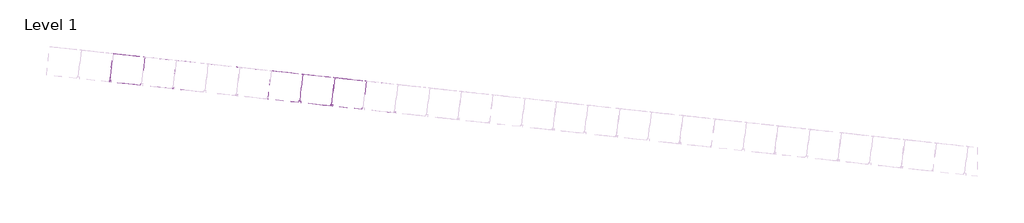
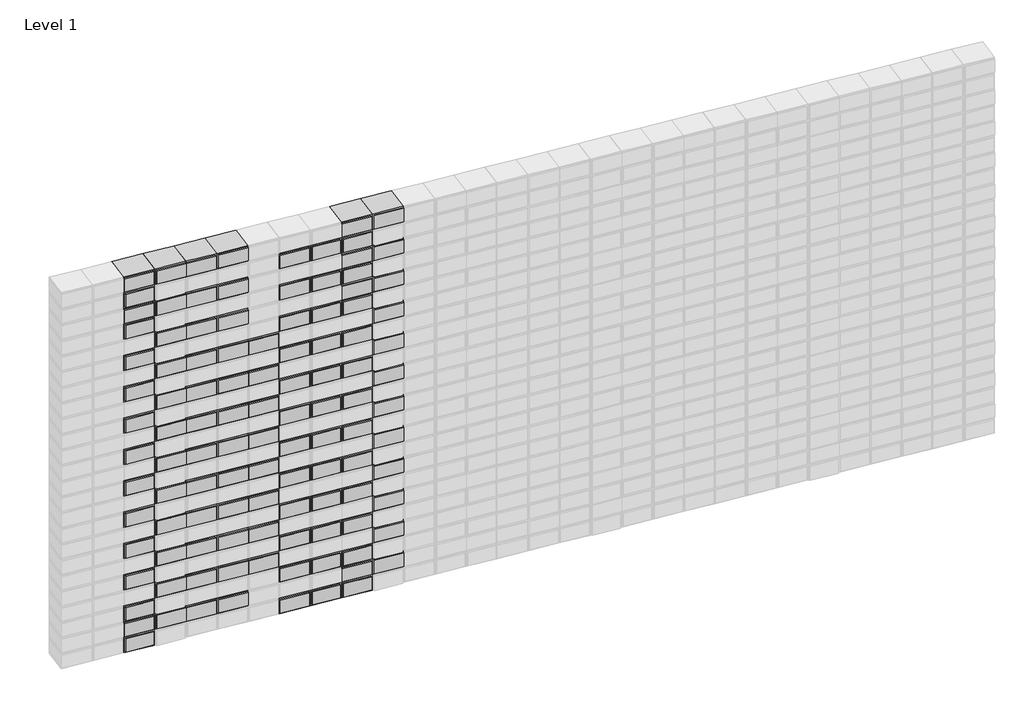
# One storey, part 12 of 18: 111 proxies.
"""IFC4 building model written with IfcOpenShell, lengths in millimetres."""

import ifcopenshell
import ifcopenshell.guid

model = None  # the IFC model being written
_history = None  # IfcOwnerHistory: only IFC2X3 demands one
_inside = {}  # id of a spatial element -> (the spatial element, [elements in it])
_under = {}  # id of a project, library or spatial element -> (it, [spatial elements below it])
_declared = {}  # id of a project -> (the project, [libraries it declares])
_typed = {}  # id of a type object -> (the type object, [elements of that type])
_made_of = {}  # id of a material, layer set ... -> (it, [elements and type objects made of it])


def new_model(schema):
    """Start an empty IFC model of exactly this schema.

    Asked for "IFC4X3", IfcOpenShell would pick the latest addendum, in which some entities
    have other attributes; the version numbers below select the first issue.
    IFC2X3 requires an IfcOwnerHistory on every rooted entity: one is made here for all.
    """
    global model, _history
    if schema == "IFC4X3":
        model = ifcopenshell.file(schema_version=(4, 3, 0, 0))
    else:
        model = ifcopenshell.file(schema=schema)
    _inside.clear()
    _under.clear()
    _declared.clear()
    _typed.clear()
    _made_of.clear()
    _history = None
    if model.schema == "IFC2X3":
        org = make("IfcOrganization", Name="unknown")
        user = make(
            "IfcPersonAndOrganization",
            ThePerson=make("IfcPerson", FamilyName="unknown"),
            TheOrganization=org,
        )
        app = make(
            "IfcApplication",
            ApplicationDeveloper=org,
            Version="unknown",
            ApplicationFullName="unknown",
            ApplicationIdentifier="unknown",
        )
        _history = make(
            "IfcOwnerHistory",
            OwningUser=user,
            OwningApplication=app,
            ChangeAction="ADDED",
            CreationDate=0,
        )
    return model


def make(cls, **values):
    """One entity of the class cls with the attributes given. An attribute that is None is left unset."""
    return model.create_entity(
        cls, **{name: value for name, value in values.items() if value is not None}
    )


def rooted(cls, **values):
    """An entity with a GlobalId (a new one), such as an element, a storey or a relation."""
    return make(cls, GlobalId=ifcopenshell.guid.new(), OwnerHistory=_history, **values)


def si_unit(unit_type, name, prefix=None):
    """IfcSIUnit, for example si_unit("LENGTHUNIT", "METRE", prefix="MILLI")."""
    return make("IfcSIUnit", UnitType=unit_type, Prefix=prefix, Name=name)


def assignment(units):
    """IfcUnitAssignment: the units of a project."""
    return None if units is None else make("IfcUnitAssignment", Units=units)


def point(xyz):
    """IfcCartesianPoint."""
    return None if xyz is None else make("IfcCartesianPoint", Coordinates=xyz)


def direction(xyz):
    """IfcDirection."""
    return None if xyz is None else make("IfcDirection", DirectionRatios=xyz)


def frame(location, z_axis=None, x_axis=None):
    """IfcAxis2Placement3D, a coordinate frame: its origin and axes. An axis left out is left unset."""
    return make(
        "IfcAxis2Placement3D",
        Location=point(location),
        Axis=direction(z_axis),
        RefDirection=direction(x_axis),
    )


def origin():
    """The frame at (0, 0, 0) with its axes left unset."""
    return frame((0.0, 0.0, 0.0))


def origin_with_axes():
    """The frame at (0, 0, 0) with the z axis (0, 0, 1) and the x axis (1, 0, 0) written out."""
    return frame((0.0, 0.0, 0.0), z_axis=(0.0, 0.0, 1.0), x_axis=(1.0, 0.0, 0.0))


def place(relative_to, where):
    """IfcLocalPlacement: puts the frame where relative to a parent placement (None: the world)."""
    return make(
        "IfcLocalPlacement", PlacementRelTo=relative_to, RelativePlacement=where
    )


def context(
    kind, dimensions, precision=None, world=None, true_north=None, identifier=None
):
    """IfcGeometricRepresentationContext, for example the 3D "Model" context."""
    return make(
        "IfcGeometricRepresentationContext",
        ContextIdentifier=identifier,
        ContextType=kind,
        CoordinateSpaceDimension=dimensions,
        Precision=precision,
        WorldCoordinateSystem=world,
        TrueNorth=true_north,
    )


def project(units=None, contexts=None):
    """IfcProject with its units and contexts."""
    return rooted(
        "IfcProject",
        Name="project",
        RepresentationContexts=contexts,
        UnitsInContext=assignment(units),
    )


def spatial(cls, under=None, at=None, **own):
    """A site, building, storey or space (cls), placed at a placement, below another one or the project."""
    s = rooted(cls, ObjectPlacement=at, **own)
    if under is not None:
        _under.setdefault(under.id(), (under, []))[1].append(s)
    return s


def polyline(points):
    """IfcPolyline through the points."""
    return make("IfcPolyline", Points=[point(p) for p in points])


def outline(outer, holes=None, kind="AREA"):
    """IfcArbitraryClosedProfileDef: a profile drawn as a closed curve; with holes, ...WithVoids."""
    if holes is None:
        return make("IfcArbitraryClosedProfileDef", ProfileType=kind, OuterCurve=outer)
    return make(
        "IfcArbitraryProfileDefWithVoids",
        ProfileType=kind,
        OuterCurve=outer,
        InnerCurves=holes,
    )


def extrude(swept, where, along, depth):
    """IfcExtrudedAreaSolid: the profile swept, set in the frame where, extruded along a direction by depth."""
    return make(
        "IfcExtrudedAreaSolid",
        SweptArea=swept,
        Position=where,
        ExtrudedDirection=direction(along),
        Depth=depth,
    )


def shape(context_of_items, identifier, shape_type, items):
    """IfcShapeRepresentation: the items that make up one representation, for example the "Body"."""
    return make(
        "IfcShapeRepresentation",
        ContextOfItems=context_of_items,
        RepresentationIdentifier=identifier,
        RepresentationType=shape_type,
        Items=items,
    )


def source(mapping_origin, context_of_items, identifier, shape_type, items):
    """IfcRepresentationMap: a shape defined once, which mapped items show again and again."""
    return make(
        "IfcRepresentationMap",
        MappingOrigin=mapping_origin,
        MappedRepresentation=shape(context_of_items, identifier, shape_type, items),
    )


def transform(
    local_origin,
    x_axis=None,
    y_axis=None,
    z_axis=None,
    scale=None,
    scale2=None,
    scale3=None,
    uniform=True,
):
    """IfcCartesianTransformationOperator3D, or its non-uniform kind. x_axis, y_axis, z_axis: its Axis1, 2, 3."""
    if uniform:
        return make(
            "IfcCartesianTransformationOperator3D",
            Axis1=direction(x_axis),
            Axis2=direction(y_axis),
            LocalOrigin=point(local_origin),
            Scale=scale,
            Axis3=direction(z_axis),
        )
    return make(
        "IfcCartesianTransformationOperator3DnonUniform",
        Axis1=direction(x_axis),
        Axis2=direction(y_axis),
        LocalOrigin=point(local_origin),
        Scale=scale,
        Axis3=direction(z_axis),
        Scale2=scale2,
        Scale3=scale3,
    )


def mapped(mapping_source, mapping_target):
    """IfcMappedItem: shows the shape of a source again, moved by a transform."""
    return make(
        "IfcMappedItem", MappingSource=mapping_source, MappingTarget=mapping_target
    )


def made_of(thing, what):
    """Note that an element or type object is made of a material, layer set ...; save() writes the relation."""
    if what is not None:
        _made_of.setdefault(what.id(), (what, []))[1].append(thing)
    return thing


def element(
    cls,
    number,
    at=None,
    inside=None,
    cuts=None,
    type_object=None,
    material=None,
    context=None,
    identifier="Body",
    shape_type=None,
    held_by="IfcProductDefinitionShape",
    body=None,
    shapes=None,
    **own,
):
    """One element of the class cls, such as IfcWall. Its Tag is "e" and its number.

    at: its placement. inside: the storey or other place that contains it. cuts: it is an
    opening in that element (IfcRelVoidsElement). A single representation is given by context,
    identifier, shape_type and body (its items); several are given by shapes. held_by: the class
    of the entity that holds the representations. save() writes the other relations.
    """
    e = rooted(cls, Tag="e%d" % number, ObjectPlacement=at, **own)
    if body is not None:
        shapes = [shape(context, identifier, shape_type, body)]
    if shapes is not None:
        e.Representation = make(held_by, Representations=shapes)
    if inside is not None:
        _inside.setdefault(inside.id(), (inside, []))[1].append(e)
    if cuts is not None:
        rooted(
            "IfcRelVoidsElement", RelatingBuildingElement=cuts, RelatedOpeningElement=e
        )
    if type_object is not None:
        _typed.setdefault(type_object.id(), (type_object, []))[1].append(e)
    return made_of(e, material)


def aggregate(whole, parts):
    """IfcRelAggregates: a whole, such as a stair, and the parts it consists of."""
    return rooted("IfcRelAggregates", RelatingObject=whole, RelatedObjects=parts)


def save(model, path):
    """Write the relations noted so far, then the file.

    IfcRelAggregates (storeys below a building ...), IfcRelContainedInSpatialStructure (elements
    in a storey), IfcRelDefinesByType, IfcRelAssociatesMaterial and IfcRelDeclares: one each for
    every whole, place, type object, material and project.
    """
    for whole, parts in _under.values():
        aggregate(whole, parts)
    for where, things in _inside.values():
        rooted(
            "IfcRelContainedInSpatialStructure",
            RelatedElements=things,
            RelatingStructure=where,
        )
    for kind, things in _typed.values():
        rooted("IfcRelDefinesByType", RelatedObjects=things, RelatingType=kind)
    for what, things in _made_of.values():
        rooted("IfcRelAssociatesMaterial", RelatedObjects=things, RelatingMaterial=what)
    for by, libraries in _declared.values():
        rooted("IfcRelDeclares", RelatingContext=by, RelatedDefinitions=libraries)
    model.write(path)


def geel_a5fc7152(model_context):
    return source(origin(), model_context, "Body", "SweptSolid", [
        extrude(outline(polyline([(131.1871262, 51.8695461), (24.8461542, 24.0369432), (23.5801491, 28.8740117), (125.0840527, 55.4406095), (111.9430518, 105.6488784), (10.4391482, 79.0822806), (9.1731432, 83.919349), (115.5141152, 111.7519519), (131.1871262, 51.8695461)])), origin_with_axes(), (0.0, 0.0, 1.0), 95.0),
        extrude(outline(polyline([(111.9430518, 105.6488784), (125.0840527, 55.4406095), (23.5801491, 28.8740117), (10.4391482, 79.0822806), (111.9430518, 105.6488784)])), origin_with_axes(), (0.0, 0.0, 1.0), 100.0),
    ])


def geel_ff5a4212(model_context):
    return source(origin(), model_context, "Body", "SweptSolid", [
        extrude(outline(polyline([(24.8461542, 24.0369432), (9.1731432, 83.919349), (115.5141152, 111.7519519), (116.7801202, 106.9148835), (15.2762167, 80.3482856), (28.4172176, 30.1400167), (129.9211211, 56.7066146), (131.1871262, 51.8695461), (24.8461542, 24.0369432)])), origin_with_axes(), (0.0, 0.0, 1.0), 95.0),
        extrude(outline(polyline([(116.7801202, 106.9148835), (129.9211211, 56.7066146), (28.4172176, 30.1400167), (15.2762167, 80.3482856), (116.7801202, 106.9148835)])), origin_with_axes(), (0.0, 0.0, 1.0), 100.0),
    ])


def rood_14a66368(model_context):
    return source(origin(), model_context, "Body", "SweptSolid", [
        extrude(outline(polyline([(24.8461542, 24.0369432), (9.1731432, 83.919349), (115.5141152, 111.7519519), (131.1871262, 51.8695461), (24.8461542, 24.0369432)]), holes=[polyline([(125.0840527, 55.4406095), (111.9430518, 105.6488784), (15.2762167, 80.3482856), (28.4172176, 30.1400167), (125.0840527, 55.4406095)])]), origin_with_axes(), (0.0, 0.0, 1.0), 95.0),
        extrude(outline(polyline([(111.9430518, 105.6488784), (125.0840527, 55.4406095), (28.4172176, 30.1400167), (15.2762167, 80.3482856), (111.9430518, 105.6488784)])), origin_with_axes(), (0.0, 0.0, 1.0), 100.0),
    ])


model = new_model("IFC4")

# Units and contexts
model_context = context("Model", 3, world=origin())
ifc_project = project(units=[si_unit("LENGTHUNIT", "METRE", prefix="MILLI")], contexts=[model_context])

# Site, building, storey
site = spatial("IfcSite", under=ifc_project)
building = spatial("IfcBuilding", under=site)
storey = spatial("IfcBuildingStorey", under=building, Name="Level 1", Elevation=0.0)

# Proxies
placement = place(None, origin())
geel_shape = geel_a5fc7152(model_context)
element("IfcBuildingElementProxy", 1, Name="Geel", ObjectType="Geel", at=placement, inside=storey, context=model_context, shape_type="MappedRepresentation", body=[
    mapped(geel_shape, transform((9860.5813726, -4383.3697112, 3159.1275502), x_axis=(0.9617275503729372, -0.1047347566147745, -0.2532010063378768), y_axis=(0.2517127736886921, -0.02741220845643024, 0.9674136914420256), z_axis=(-0.10826263628609285, -0.9941223272738547, 0.0))),
])
element("IfcBuildingElementProxy", 2, Name="Geel", ObjectType="Geel", at=placement, inside=storey, context=model_context, shape_type="MappedRepresentation", body=[
    mapped(geel_shape, transform((9095.6433234, -4300.0658686, 3282.926513), x_axis=(0.9617275503729401, -0.10473475661476903, -0.2532010063378687), y_axis=(0.2517127736886843, -0.02741220845642789, 0.9674136914420278), z_axis=(-0.108262636286087, -0.9941223272738555, 0.0))),
])
element("IfcBuildingElementProxy", 3, Name="Geel", ObjectType="Geel", at=placement, inside=storey, context=model_context, shape_type="MappedRepresentation", body=[
    mapped(geel_shape, transform((9860.5813726, -4383.3697112, 3282.926513), x_axis=(0.9617275503729372, -0.1047347566147745, -0.2532010063378768), y_axis=(0.2517127736886921, -0.02741220845643024, 0.9674136914420256), z_axis=(-0.10826263628609285, -0.9941223272738547, 0.0))),
])
element("IfcBuildingElementProxy", 4, Name="Geel", ObjectType="Geel", at=placement, inside=storey, context=model_context, shape_type="MappedRepresentation", body=[
    mapped(geel_shape, transform((9095.6433234, -4300.0658686, 3406.7254759), x_axis=(0.9617275503729401, -0.10473475661476903, -0.2532010063378687), y_axis=(0.2517127736886843, -0.02741220845642789, 0.9674136914420278), z_axis=(-0.108262636286087, -0.9941223272738555, 0.0))),
])
element("IfcBuildingElementProxy", 5, Name="Geel", ObjectType="Geel", at=placement, inside=storey, context=model_context, shape_type="MappedRepresentation", body=[
    mapped(geel_shape, transform((9860.5813726, -4383.3697112, 3406.7254759), x_axis=(0.9617275503729372, -0.1047347566147745, -0.2532010063378768), y_axis=(0.2517127736886921, -0.02741220845643024, 0.9674136914420256), z_axis=(-0.10826263628609285, -0.9941223272738547, 0.0))),
])
element("IfcBuildingElementProxy", 6, Name="Geel", ObjectType="Geel", at=placement, inside=storey, context=model_context, shape_type="MappedRepresentation", body=[
    mapped(geel_shape, transform((9095.6433234, -4300.0658686, 2044.9368847), x_axis=(0.961727550372941, -0.10473475661476911, -0.2532010063378651), y_axis=(0.2517127736886807, -0.0274122084564275, 0.9674136914420286), z_axis=(-0.10826263628608698, -0.9941223272738555, 0.0))),
])
element("IfcBuildingElementProxy", 7, Name="Geel", ObjectType="Geel", at=placement, inside=storey, context=model_context, shape_type="MappedRepresentation", body=[
    mapped(geel_shape, transform((9860.5813726, -4383.3697112, 2044.9368847), x_axis=(0.9617275503729381, -0.10473475661477456, -0.2532010063378731), y_axis=(0.2517127736886886, -0.02741220845642988, 0.9674136914420264), z_axis=(-0.10826263628609287, -0.9941223272738549, 0.0))),
])
element("IfcBuildingElementProxy", 8, Name="Geel", ObjectType="Geel", at=placement, inside=storey, context=model_context, shape_type="MappedRepresentation", body=[
    mapped(geel_shape, transform((9314.1970517, -4323.8669665, 2168.7358475), x_axis=(0.9617275503729396, -0.10473475661477374, -0.25320100633786874), y_axis=(0.251712773688684, -0.027412208456429103, 0.9674136914420278), z_axis=(-0.10826263628609185, -0.994122327273855, 0.0))),
])
element("IfcBuildingElementProxy", 9, Name="Geel", ObjectType="Geel", at=placement, inside=storey, context=model_context, shape_type="MappedRepresentation", body=[
    mapped(geel_shape, transform((9314.1970517, -4323.8669665, 2292.5348104), x_axis=(0.9617275503729396, -0.10473475661477374, -0.25320100633786874), y_axis=(0.251712773688684, -0.027412208456429103, 0.9674136914420278), z_axis=(-0.10826263628609185, -0.994122327273855, 0.0))),
])
element("IfcBuildingElementProxy", 10, Name="Geel", ObjectType="Geel", at=placement, inside=storey, context=model_context, shape_type="MappedRepresentation", body=[
    mapped(geel_shape, transform((9314.1970517, -4323.8669665, 2416.3337732), x_axis=(0.9617275503729403, -0.10473475661477383, -0.253201006337865), y_axis=(0.2517127736886804, -0.0274122084564287, 0.9674136914420286), z_axis=(-0.10826263628609184, -0.9941223272738549, 0.0))),
])
element("IfcBuildingElementProxy", 11, Name="Geel", ObjectType="Geel", at=placement, inside=storey, context=model_context, shape_type="MappedRepresentation", body=[
    mapped(geel_shape, transform((9314.1970517, -4323.8669665, 2540.132736), x_axis=(0.9617275503729396, -0.10473475661477374, -0.25320100633786874), y_axis=(0.251712773688684, -0.027412208456429103, 0.9674136914420278), z_axis=(-0.10826263628609185, -0.994122327273855, 0.0))),
])
element("IfcBuildingElementProxy", 12, Name="Geel", ObjectType="Geel", at=placement, inside=storey, context=model_context, shape_type="MappedRepresentation", body=[
    mapped(geel_shape, transform((9314.1970517, -4323.8669665, 2663.9316989), x_axis=(0.9617275503729396, -0.10473475661477374, -0.25320100633786874), y_axis=(0.251712773688684, -0.027412208456429103, 0.9674136914420278), z_axis=(-0.10826263628609185, -0.994122327273855, 0.0))),
])
element("IfcBuildingElementProxy", 13, Name="Geel", ObjectType="Geel", at=placement, inside=storey, context=model_context, shape_type="MappedRepresentation", body=[
    mapped(geel_shape, transform((9314.1970517, -4323.8669665, 2787.7306617), x_axis=(0.9617275503729396, -0.10473475661477374, -0.25320100633786874), y_axis=(0.251712773688684, -0.027412208456429103, 0.9674136914420278), z_axis=(-0.10826263628609185, -0.994122327273855, 0.0))),
])
element("IfcBuildingElementProxy", 14, Name="Geel", ObjectType="Geel", at=placement, inside=storey, context=model_context, shape_type="MappedRepresentation", body=[
    mapped(geel_shape, transform((9314.1970517, -4323.8669665, 2911.5296245), x_axis=(0.9617275503729396, -0.10473475661477374, -0.25320100633786874), y_axis=(0.251712773688684, -0.027412208456429103, 0.9674136914420278), z_axis=(-0.10826263628609185, -0.994122327273855, 0.0))),
])
element("IfcBuildingElementProxy", 15, Name="Geel", ObjectType="Geel", at=placement, inside=storey, context=model_context, shape_type="MappedRepresentation", body=[
    mapped(geel_shape, transform((9314.1970517, -4323.8669665, 3035.3285874), x_axis=(0.9617275503729396, -0.10473475661477374, -0.25320100633786874), y_axis=(0.251712773688684, -0.027412208456429103, 0.9674136914420278), z_axis=(-0.10826263628609185, -0.994122327273855, 0.0))),
])
element("IfcBuildingElementProxy", 16, Name="Geel", ObjectType="Geel", at=placement, inside=storey, context=model_context, shape_type="MappedRepresentation", body=[
    mapped(geel_shape, transform((9314.1970517, -4323.8669665, 3159.1275502), x_axis=(0.9617275503729396, -0.10473475661477374, -0.25320100633786874), y_axis=(0.251712773688684, -0.027412208456429103, 0.9674136914420278), z_axis=(-0.10826263628609185, -0.994122327273855, 0.0))),
])
element("IfcBuildingElementProxy", 17, Name="Geel", ObjectType="Geel", at=placement, inside=storey, context=model_context, shape_type="MappedRepresentation", body=[
    mapped(geel_shape, transform((9314.1970517, -4323.8669665, 3282.926513), x_axis=(0.9617275503729396, -0.10473475661477374, -0.25320100633786874), y_axis=(0.251712773688684, -0.027412208456429103, 0.9674136914420278), z_axis=(-0.10826263628609185, -0.994122327273855, 0.0))),
])
element("IfcBuildingElementProxy", 18, Name="Geel", ObjectType="Geel", at=placement, inside=storey, context=model_context, shape_type="MappedRepresentation", body=[
    mapped(geel_shape, transform((9314.1970517, -4323.8669665, 3406.7254759), x_axis=(0.9617275503729396, -0.10473475661477374, -0.25320100633786874), y_axis=(0.251712773688684, -0.027412208456429103, 0.9674136914420278), z_axis=(-0.10826263628609185, -0.994122327273855, 0.0))),
])
element("IfcBuildingElementProxy", 19, Name="Geel", ObjectType="Geel", at=placement, inside=storey, context=model_context, shape_type="MappedRepresentation", body=[
    mapped(geel_shape, transform((9314.1970517, -4323.8669665, 2044.9368847), x_axis=(0.9617275503729403, -0.10473475661477383, -0.253201006337865), y_axis=(0.2517127736886804, -0.0274122084564287, 0.9674136914420286), z_axis=(-0.10826263628609184, -0.9941223272738549, 0.0))),
])
element("IfcBuildingElementProxy", 20, Name="Geel", ObjectType="Geel", at=placement, inside=storey, context=model_context, shape_type="MappedRepresentation", body=[
    mapped(geel_shape, transform((9532.7507801, -4347.6680644, 2168.7358475), x_axis=(0.9617275503729374, -0.1047347566147725, -0.25320100633787673), y_axis=(0.25171277368869216, -0.02741220845642974, 0.9674136914420255), z_axis=(-0.10826263628609081, -0.9941223272738551, 0.0))),
])
element("IfcBuildingElementProxy", 21, Name="Geel", ObjectType="Geel", at=placement, inside=storey, context=model_context, shape_type="MappedRepresentation", body=[
    mapped(geel_shape, transform((9532.7507801, -4347.6680644, 2292.5348104), x_axis=(0.9617275503729374, -0.1047347566147725, -0.25320100633787673), y_axis=(0.25171277368869216, -0.02741220845642974, 0.9674136914420255), z_axis=(-0.10826263628609081, -0.9941223272738551, 0.0))),
])
element("IfcBuildingElementProxy", 22, Name="Geel", ObjectType="Geel", at=placement, inside=storey, context=model_context, shape_type="MappedRepresentation", body=[
    mapped(geel_shape, transform((9532.7507801, -4347.6680644, 2416.3337732), x_axis=(0.9617275503729384, -0.1047347566147726, -0.25320100633787307), y_axis=(0.25171277368868855, -0.02741220845642934, 0.9674136914420265), z_axis=(-0.10826263628609081, -0.994122327273855, 0.0))),
])
element("IfcBuildingElementProxy", 23, Name="Geel", ObjectType="Geel", at=placement, inside=storey, context=model_context, shape_type="MappedRepresentation", body=[
    mapped(geel_shape, transform((9532.7507801, -4347.6680644, 2540.132736), x_axis=(0.9617275503729374, -0.1047347566147725, -0.25320100633787673), y_axis=(0.25171277368869216, -0.02741220845642974, 0.9674136914420255), z_axis=(-0.10826263628609081, -0.9941223272738551, 0.0))),
])
element("IfcBuildingElementProxy", 24, Name="Geel", ObjectType="Geel", at=placement, inside=storey, context=model_context, shape_type="MappedRepresentation", body=[
    mapped(geel_shape, transform((9532.7507801, -4347.6680644, 2663.9316989), x_axis=(0.9617275503729374, -0.1047347566147725, -0.25320100633787673), y_axis=(0.25171277368869216, -0.02741220845642974, 0.9674136914420255), z_axis=(-0.10826263628609081, -0.9941223272738551, 0.0))),
])
element("IfcBuildingElementProxy", 25, Name="Geel", ObjectType="Geel", at=placement, inside=storey, context=model_context, shape_type="MappedRepresentation", body=[
    mapped(geel_shape, transform((9532.7507801, -4347.6680644, 2787.7306617), x_axis=(0.9617275503729374, -0.1047347566147725, -0.25320100633787673), y_axis=(0.25171277368869216, -0.02741220845642974, 0.9674136914420255), z_axis=(-0.10826263628609081, -0.9941223272738551, 0.0))),
])
element("IfcBuildingElementProxy", 26, Name="Geel", ObjectType="Geel", at=placement, inside=storey, context=model_context, shape_type="MappedRepresentation", body=[
    mapped(geel_shape, transform((9532.7507801, -4347.6680644, 2911.5296245), x_axis=(0.9617275503729374, -0.1047347566147725, -0.25320100633787673), y_axis=(0.25171277368869216, -0.02741220845642974, 0.9674136914420255), z_axis=(-0.10826263628609081, -0.9941223272738551, 0.0))),
])
element("IfcBuildingElementProxy", 27, Name="Geel", ObjectType="Geel", at=placement, inside=storey, context=model_context, shape_type="MappedRepresentation", body=[
    mapped(geel_shape, transform((9532.7507801, -4347.6680644, 3035.3285874), x_axis=(0.9617275503729374, -0.1047347566147725, -0.25320100633787673), y_axis=(0.25171277368869216, -0.02741220845642974, 0.9674136914420255), z_axis=(-0.10826263628609081, -0.9941223272738551, 0.0))),
])
geel_2_shape = geel_ff5a4212(model_context)
element("IfcBuildingElementProxy", 28, Name="Geel", ObjectType="Geel", at=placement, inside=storey, context=model_context, shape_type="MappedRepresentation", body=[
    mapped(geel_2_shape, transform((9204.9201876, -4311.9664176, 2168.7358475), x_axis=(0.9617275503729374, -0.1047347566147725, -0.25320100633787673), y_axis=(0.25171277368869216, -0.02741220845642974, 0.9674136914420255), z_axis=(-0.10826263628609081, -0.9941223272738551, 0.0))),
])
element("IfcBuildingElementProxy", 29, Name="Geel", ObjectType="Geel", at=placement, inside=storey, context=model_context, shape_type="MappedRepresentation", body=[
    mapped(geel_2_shape, transform((9969.8582368, -4395.2702601, 2168.7358475), x_axis=(0.9617275503729374, -0.1047347566147725, -0.25320100633787673), y_axis=(0.25171277368869216, -0.02741220845642974, 0.9674136914420255), z_axis=(-0.10826263628609081, -0.9941223272738551, 0.0))),
])
element("IfcBuildingElementProxy", 30, Name="Geel", ObjectType="Geel", at=placement, inside=storey, context=model_context, shape_type="MappedRepresentation", body=[
    mapped(geel_2_shape, transform((9204.9201876, -4311.9664176, 2292.5348104), x_axis=(0.9617275503729374, -0.1047347566147725, -0.25320100633787673), y_axis=(0.25171277368869216, -0.02741220845642974, 0.9674136914420255), z_axis=(-0.10826263628609081, -0.9941223272738551, 0.0))),
])
element("IfcBuildingElementProxy", 31, Name="Geel", ObjectType="Geel", at=placement, inside=storey, context=model_context, shape_type="MappedRepresentation", body=[
    mapped(geel_2_shape, transform((9969.8582368, -4395.2702601, 2292.5348104), x_axis=(0.9617275503729374, -0.1047347566147725, -0.25320100633787673), y_axis=(0.25171277368869216, -0.02741220845642974, 0.9674136914420255), z_axis=(-0.10826263628609081, -0.9941223272738551, 0.0))),
])
element("IfcBuildingElementProxy", 32, Name="Geel", ObjectType="Geel", at=placement, inside=storey, context=model_context, shape_type="MappedRepresentation", body=[
    mapped(geel_2_shape, transform((9204.9201876, -4311.9664176, 2416.3337732), x_axis=(0.9617275503729384, -0.1047347566147726, -0.25320100633787307), y_axis=(0.25171277368868855, -0.02741220845642934, 0.9674136914420265), z_axis=(-0.10826263628609081, -0.994122327273855, 0.0))),
])
element("IfcBuildingElementProxy", 33, Name="Geel", ObjectType="Geel", at=placement, inside=storey, context=model_context, shape_type="MappedRepresentation", body=[
    mapped(geel_2_shape, transform((9969.8582368, -4395.2702601, 2416.3337732), x_axis=(0.9617275503729384, -0.1047347566147726, -0.25320100633787307), y_axis=(0.25171277368868855, -0.02741220845642934, 0.9674136914420265), z_axis=(-0.10826263628609081, -0.994122327273855, 0.0))),
])
element("IfcBuildingElementProxy", 34, Name="Geel", ObjectType="Geel", at=placement, inside=storey, context=model_context, shape_type="MappedRepresentation", body=[
    mapped(geel_2_shape, transform((9204.9201876, -4311.9664176, 2540.132736), x_axis=(0.9617275503729374, -0.1047347566147725, -0.25320100633787673), y_axis=(0.25171277368869216, -0.02741220845642974, 0.9674136914420255), z_axis=(-0.10826263628609081, -0.9941223272738551, 0.0))),
])
element("IfcBuildingElementProxy", 35, Name="Geel", ObjectType="Geel", at=placement, inside=storey, context=model_context, shape_type="MappedRepresentation", body=[
    mapped(geel_2_shape, transform((9969.8582368, -4395.2702601, 2540.132736), x_axis=(0.9617275503729374, -0.1047347566147725, -0.25320100633787673), y_axis=(0.25171277368869216, -0.02741220845642974, 0.9674136914420255), z_axis=(-0.10826263628609081, -0.9941223272738551, 0.0))),
])
element("IfcBuildingElementProxy", 36, Name="Geel", ObjectType="Geel", at=placement, inside=storey, context=model_context, shape_type="MappedRepresentation", body=[
    mapped(geel_2_shape, transform((9204.9201876, -4311.9664176, 2663.9316989), x_axis=(0.9617275503729374, -0.1047347566147725, -0.25320100633787673), y_axis=(0.25171277368869216, -0.02741220845642974, 0.9674136914420255), z_axis=(-0.10826263628609081, -0.9941223272738551, 0.0))),
])
element("IfcBuildingElementProxy", 37, Name="Geel", ObjectType="Geel", at=placement, inside=storey, context=model_context, shape_type="MappedRepresentation", body=[
    mapped(geel_2_shape, transform((9969.8582368, -4395.2702601, 2663.9316989), x_axis=(0.9617275503729374, -0.1047347566147725, -0.25320100633787673), y_axis=(0.25171277368869216, -0.02741220845642974, 0.9674136914420255), z_axis=(-0.10826263628609081, -0.9941223272738551, 0.0))),
])
element("IfcBuildingElementProxy", 38, Name="Geel", ObjectType="Geel", at=placement, inside=storey, context=model_context, shape_type="MappedRepresentation", body=[
    mapped(geel_2_shape, transform((9204.9201876, -4311.9664176, 2787.7306617), x_axis=(0.9617275503729374, -0.1047347566147725, -0.25320100633787673), y_axis=(0.25171277368869216, -0.02741220845642974, 0.9674136914420255), z_axis=(-0.10826263628609081, -0.9941223272738551, 0.0))),
])
element("IfcBuildingElementProxy", 39, Name="Geel", ObjectType="Geel", at=placement, inside=storey, context=model_context, shape_type="MappedRepresentation", body=[
    mapped(geel_2_shape, transform((9969.8582368, -4395.2702601, 2787.7306617), x_axis=(0.9617275503729374, -0.1047347566147725, -0.25320100633787673), y_axis=(0.25171277368869216, -0.02741220845642974, 0.9674136914420255), z_axis=(-0.10826263628609081, -0.9941223272738551, 0.0))),
])
element("IfcBuildingElementProxy", 40, Name="Geel", ObjectType="Geel", at=placement, inside=storey, context=model_context, shape_type="MappedRepresentation", body=[
    mapped(geel_2_shape, transform((9204.9201876, -4311.9664176, 2911.5296245), x_axis=(0.9617275503729374, -0.1047347566147725, -0.25320100633787673), y_axis=(0.25171277368869216, -0.02741220845642974, 0.9674136914420255), z_axis=(-0.10826263628609081, -0.9941223272738551, 0.0))),
])
element("IfcBuildingElementProxy", 41, Name="Geel", ObjectType="Geel", at=placement, inside=storey, context=model_context, shape_type="MappedRepresentation", body=[
    mapped(geel_2_shape, transform((9969.8582368, -4395.2702601, 2911.5296245), x_axis=(0.9617275503729374, -0.1047347566147725, -0.25320100633787673), y_axis=(0.25171277368869216, -0.02741220845642974, 0.9674136914420255), z_axis=(-0.10826263628609081, -0.9941223272738551, 0.0))),
])
element("IfcBuildingElementProxy", 42, Name="Geel", ObjectType="Geel", at=placement, inside=storey, context=model_context, shape_type="MappedRepresentation", body=[
    mapped(geel_2_shape, transform((9204.9201876, -4311.9664176, 3035.3285874), x_axis=(0.9617275503729374, -0.1047347566147725, -0.25320100633787673), y_axis=(0.25171277368869216, -0.02741220845642974, 0.9674136914420255), z_axis=(-0.10826263628609081, -0.9941223272738551, 0.0))),
])
element("IfcBuildingElementProxy", 43, Name="Geel", ObjectType="Geel", at=placement, inside=storey, context=model_context, shape_type="MappedRepresentation", body=[
    mapped(geel_2_shape, transform((9969.8582368, -4395.2702601, 3035.3285874), x_axis=(0.9617275503729374, -0.1047347566147725, -0.25320100633787673), y_axis=(0.25171277368869216, -0.02741220845642974, 0.9674136914420255), z_axis=(-0.10826263628609081, -0.9941223272738551, 0.0))),
])
element("IfcBuildingElementProxy", 44, Name="Geel", ObjectType="Geel", at=placement, inside=storey, context=model_context, shape_type="MappedRepresentation", body=[
    mapped(geel_2_shape, transform((9204.9201876, -4311.9664176, 3159.1275502), x_axis=(0.9617275503729374, -0.1047347566147725, -0.25320100633787673), y_axis=(0.25171277368869216, -0.02741220845642974, 0.9674136914420255), z_axis=(-0.10826263628609081, -0.9941223272738551, 0.0))),
])
element("IfcBuildingElementProxy", 45, Name="Geel", ObjectType="Geel", at=placement, inside=storey, context=model_context, shape_type="MappedRepresentation", body=[
    mapped(geel_2_shape, transform((9969.8582368, -4395.2702601, 3159.1275502), x_axis=(0.9617275503729374, -0.1047347566147725, -0.25320100633787673), y_axis=(0.25171277368869216, -0.02741220845642974, 0.9674136914420255), z_axis=(-0.10826263628609081, -0.9941223272738551, 0.0))),
])
element("IfcBuildingElementProxy", 46, Name="Geel", ObjectType="Geel", at=placement, inside=storey, context=model_context, shape_type="MappedRepresentation", body=[
    mapped(geel_2_shape, transform((9204.9201876, -4311.9664176, 3282.926513), x_axis=(0.9617275503729374, -0.1047347566147725, -0.25320100633787673), y_axis=(0.25171277368869216, -0.02741220845642974, 0.9674136914420255), z_axis=(-0.10826263628609081, -0.9941223272738551, 0.0))),
])
element("IfcBuildingElementProxy", 47, Name="Geel", ObjectType="Geel", at=placement, inside=storey, context=model_context, shape_type="MappedRepresentation", body=[
    mapped(geel_2_shape, transform((9969.8582368, -4395.2702601, 3282.926513), x_axis=(0.9617275503729374, -0.1047347566147725, -0.25320100633787673), y_axis=(0.25171277368869216, -0.02741220845642974, 0.9674136914420255), z_axis=(-0.10826263628609081, -0.9941223272738551, 0.0))),
])
element("IfcBuildingElementProxy", 48, Name="Geel", ObjectType="Geel", at=placement, inside=storey, context=model_context, shape_type="MappedRepresentation", body=[
    mapped(geel_2_shape, transform((9204.9201876, -4311.9664176, 3406.7254759), x_axis=(0.9617275503729374, -0.1047347566147725, -0.25320100633787673), y_axis=(0.25171277368869216, -0.02741220845642974, 0.9674136914420255), z_axis=(-0.10826263628609081, -0.9941223272738551, 0.0))),
])
element("IfcBuildingElementProxy", 49, Name="Geel", ObjectType="Geel", at=placement, inside=storey, context=model_context, shape_type="MappedRepresentation", body=[
    mapped(geel_2_shape, transform((9969.8582368, -4395.2702601, 3406.7254759), x_axis=(0.9617275503729374, -0.1047347566147725, -0.25320100633787673), y_axis=(0.25171277368869216, -0.02741220845642974, 0.9674136914420255), z_axis=(-0.10826263628609081, -0.9941223272738551, 0.0))),
])
element("IfcBuildingElementProxy", 50, Name="Geel", ObjectType="Geel", at=placement, inside=storey, context=model_context, shape_type="MappedRepresentation", body=[
    mapped(geel_2_shape, transform((9204.9201876, -4311.9664176, 2044.9368847), x_axis=(0.9617275503729384, -0.1047347566147726, -0.25320100633787307), y_axis=(0.25171277368868855, -0.02741220845642934, 0.9674136914420265), z_axis=(-0.10826263628609081, -0.994122327273855, 0.0))),
])
element("IfcBuildingElementProxy", 51, Name="Geel", ObjectType="Geel", at=placement, inside=storey, context=model_context, shape_type="MappedRepresentation", body=[
    mapped(geel_2_shape, transform((9969.8582368, -4395.2702601, 2044.9368847), x_axis=(0.9617275503729384, -0.1047347566147726, -0.25320100633787307), y_axis=(0.25171277368868855, -0.02741220845642934, 0.9674136914420265), z_axis=(-0.10826263628609081, -0.994122327273855, 0.0))),
])
element("IfcBuildingElementProxy", 52, Name="Geel", ObjectType="Geel", at=placement, inside=storey, context=model_context, shape_type="MappedRepresentation", body=[
    mapped(geel_2_shape, transform((9423.4739159, -4335.7675154, 2168.7358475), x_axis=(0.9617275503729402, -0.10473475661476898, -0.2532010063378681), y_axis=(0.25171277368868383, -0.02741220845642784, 0.9674136914420278), z_axis=(-0.10826263628608696, -0.9941223272738555, 0.0))),
])
element("IfcBuildingElementProxy", 53, Name="Geel", ObjectType="Geel", at=placement, inside=storey, context=model_context, shape_type="MappedRepresentation", body=[
    mapped(geel_2_shape, transform((9423.4739159, -4335.7675154, 2292.5348104), x_axis=(0.9617275503729402, -0.10473475661476898, -0.2532010063378681), y_axis=(0.25171277368868383, -0.02741220845642784, 0.9674136914420278), z_axis=(-0.10826263628608696, -0.9941223272738555, 0.0))),
])
element("IfcBuildingElementProxy", 54, Name="Geel", ObjectType="Geel", at=placement, inside=storey, context=model_context, shape_type="MappedRepresentation", body=[
    mapped(geel_2_shape, transform((9423.4739159, -4335.7675154, 2416.3337732), x_axis=(0.9617275503729411, -0.10473475661476908, -0.2532010063378646), y_axis=(0.25171277368868017, -0.027412208456427424, 0.9674136914420287), z_axis=(-0.10826263628608693, -0.9941223272738554, 0.0))),
])
element("IfcBuildingElementProxy", 55, Name="Geel", ObjectType="Geel", at=placement, inside=storey, context=model_context, shape_type="MappedRepresentation", body=[
    mapped(geel_2_shape, transform((9423.4739159, -4335.7675154, 2540.132736), x_axis=(0.9617275503729402, -0.10473475661476898, -0.2532010063378681), y_axis=(0.25171277368868383, -0.02741220845642784, 0.9674136914420278), z_axis=(-0.10826263628608696, -0.9941223272738555, 0.0))),
])
element("IfcBuildingElementProxy", 56, Name="Geel", ObjectType="Geel", at=placement, inside=storey, context=model_context, shape_type="MappedRepresentation", body=[
    mapped(geel_2_shape, transform((9423.4739159, -4335.7675154, 2663.9316989), x_axis=(0.9617275503729402, -0.10473475661476898, -0.2532010063378681), y_axis=(0.25171277368868383, -0.02741220845642784, 0.9674136914420278), z_axis=(-0.10826263628608696, -0.9941223272738555, 0.0))),
])
element("IfcBuildingElementProxy", 57, Name="Geel", ObjectType="Geel", at=placement, inside=storey, context=model_context, shape_type="MappedRepresentation", body=[
    mapped(geel_2_shape, transform((9423.4739159, -4335.7675154, 2787.7306617), x_axis=(0.9617275503729402, -0.10473475661476898, -0.2532010063378681), y_axis=(0.25171277368868383, -0.02741220845642784, 0.9674136914420278), z_axis=(-0.10826263628608696, -0.9941223272738555, 0.0))),
])
element("IfcBuildingElementProxy", 58, Name="Geel", ObjectType="Geel", at=placement, inside=storey, context=model_context, shape_type="MappedRepresentation", body=[
    mapped(geel_2_shape, transform((9423.4739159, -4335.7675154, 2911.5296245), x_axis=(0.9617275503729402, -0.10473475661476898, -0.2532010063378681), y_axis=(0.25171277368868383, -0.02741220845642784, 0.9674136914420278), z_axis=(-0.10826263628608696, -0.9941223272738555, 0.0))),
])
element("IfcBuildingElementProxy", 59, Name="Geel", ObjectType="Geel", at=placement, inside=storey, context=model_context, shape_type="MappedRepresentation", body=[
    mapped(geel_2_shape, transform((9423.4739159, -4335.7675154, 3035.3285874), x_axis=(0.9617275503729402, -0.10473475661476898, -0.2532010063378681), y_axis=(0.25171277368868383, -0.02741220845642784, 0.9674136914420278), z_axis=(-0.10826263628608696, -0.9941223272738555, 0.0))),
])
element("IfcBuildingElementProxy", 60, Name="Geel", ObjectType="Geel", at=placement, inside=storey, context=model_context, shape_type="MappedRepresentation", body=[
    mapped(geel_2_shape, transform((9423.4739159, -4335.7675154, 3159.1275502), x_axis=(0.9617275503729402, -0.10473475661476898, -0.2532010063378681), y_axis=(0.25171277368868383, -0.02741220845642784, 0.9674136914420278), z_axis=(-0.10826263628608696, -0.9941223272738555, 0.0))),
])
element("IfcBuildingElementProxy", 61, Name="Geel", ObjectType="Geel", at=placement, inside=storey, context=model_context, shape_type="MappedRepresentation", body=[
    mapped(geel_2_shape, transform((9423.4739159, -4335.7675154, 3282.926513), x_axis=(0.9617275503729402, -0.10473475661476898, -0.2532010063378681), y_axis=(0.25171277368868383, -0.02741220845642784, 0.9674136914420278), z_axis=(-0.10826263628608696, -0.9941223272738555, 0.0))),
])
element("IfcBuildingElementProxy", 62, Name="Geel", ObjectType="Geel", at=placement, inside=storey, context=model_context, shape_type="MappedRepresentation", body=[
    mapped(geel_2_shape, transform((9423.4739159, -4335.7675154, 3406.7254759), x_axis=(0.9617275503729402, -0.10473475661476898, -0.2532010063378681), y_axis=(0.25171277368868383, -0.02741220845642784, 0.9674136914420278), z_axis=(-0.10826263628608696, -0.9941223272738555, 0.0))),
])
element("IfcBuildingElementProxy", 63, Name="Geel", ObjectType="Geel", at=placement, inside=storey, context=model_context, shape_type="MappedRepresentation", body=[
    mapped(geel_2_shape, transform((9423.4739159, -4335.7675154, 2044.9368847), x_axis=(0.9617275503729411, -0.10473475661476908, -0.2532010063378646), y_axis=(0.25171277368868017, -0.027412208456427424, 0.9674136914420287), z_axis=(-0.10826263628608693, -0.9941223272738554, 0.0))),
])
element("IfcBuildingElementProxy", 64, Name="Rood", ObjectType="Rood", at=placement, inside=storey, context=model_context, shape_type="MappedRepresentation", body=[
    mapped(geel_shape, transform((9642.0276443, -4359.5686133, 2106.8363661), x_axis=(0.9617275503729374, -0.1047347566147725, -0.25320100633787673), y_axis=(0.25171277368869216, -0.02741220845642974, 0.9674136914420255), z_axis=(-0.10826263628609081, -0.9941223272738551, 0.0))),
])
element("IfcBuildingElementProxy", 65, Name="Rood", ObjectType="Rood", at=placement, inside=storey, context=model_context, shape_type="MappedRepresentation", body=[
    mapped(geel_shape, transform((9642.0276443, -4359.5686133, 2230.6353289), x_axis=(0.9617275503729384, -0.1047347566147726, -0.25320100633787307), y_axis=(0.25171277368868855, -0.02741220845642934, 0.9674136914420265), z_axis=(-0.10826263628609081, -0.994122327273855, 0.0))),
])
element("IfcBuildingElementProxy", 66, Name="Rood", ObjectType="Rood", at=placement, inside=storey, context=model_context, shape_type="MappedRepresentation", body=[
    mapped(geel_shape, transform((9642.0276443, -4359.5686133, 2354.4342918), x_axis=(0.9617275503729374, -0.1047347566147725, -0.25320100633787673), y_axis=(0.25171277368869216, -0.02741220845642974, 0.9674136914420255), z_axis=(-0.10826263628609081, -0.9941223272738551, 0.0))),
])
element("IfcBuildingElementProxy", 67, Name="Rood", ObjectType="Rood", at=placement, inside=storey, context=model_context, shape_type="MappedRepresentation", body=[
    mapped(geel_shape, transform((9642.0276443, -4359.5686133, 2478.2332546), x_axis=(0.9617275503729374, -0.1047347566147725, -0.25320100633787673), y_axis=(0.25171277368869216, -0.02741220845642974, 0.9674136914420255), z_axis=(-0.10826263628609081, -0.9941223272738551, 0.0))),
])
element("IfcBuildingElementProxy", 68, Name="Rood", ObjectType="Rood", at=placement, inside=storey, context=model_context, shape_type="MappedRepresentation", body=[
    mapped(geel_shape, transform((9642.0276443, -4359.5686133, 2602.0322174), x_axis=(0.9617275503729394, -0.10473475661477268, -0.2532010063378695), y_axis=(0.2517127736886849, -0.027412208456428923, 0.9674136914420275), z_axis=(-0.1082626362860908, -0.9941223272738551, 0.0))),
])
element("IfcBuildingElementProxy", 69, Name="Rood", ObjectType="Rood", at=placement, inside=storey, context=model_context, shape_type="MappedRepresentation", body=[
    mapped(geel_shape, transform((9642.0276443, -4359.5686133, 2725.8311803), x_axis=(0.9617275503729374, -0.1047347566147725, -0.25320100633787673), y_axis=(0.25171277368869216, -0.02741220845642974, 0.9674136914420255), z_axis=(-0.10826263628609081, -0.9941223272738551, 0.0))),
])
element("IfcBuildingElementProxy", 70, Name="Rood", ObjectType="Rood", at=placement, inside=storey, context=model_context, shape_type="MappedRepresentation", body=[
    mapped(geel_shape, transform((9642.0276443, -4359.5686133, 2849.6301431), x_axis=(0.9617275503729374, -0.1047347566147725, -0.25320100633787673), y_axis=(0.25171277368869216, -0.02741220845642974, 0.9674136914420255), z_axis=(-0.10826263628609081, -0.9941223272738551, 0.0))),
])
element("IfcBuildingElementProxy", 71, Name="Rood", ObjectType="Rood", at=placement, inside=storey, context=model_context, shape_type="MappedRepresentation", body=[
    mapped(geel_shape, transform((9642.0276443, -4359.5686133, 2973.4291059), x_axis=(0.9617275503729374, -0.1047347566147725, -0.25320100633787673), y_axis=(0.25171277368869216, -0.02741220845642974, 0.9674136914420255), z_axis=(-0.10826263628609081, -0.9941223272738551, 0.0))),
])
element("IfcBuildingElementProxy", 72, Name="Rood", ObjectType="Rood", at=placement, inside=storey, context=model_context, shape_type="MappedRepresentation", body=[
    mapped(geel_shape, transform((9642.0276443, -4359.5686133, 3097.2280688), x_axis=(0.9617275503729394, -0.10473475661477268, -0.2532010063378695), y_axis=(0.2517127736886849, -0.027412208456428923, 0.9674136914420275), z_axis=(-0.1082626362860908, -0.9941223272738551, 0.0))),
])
element("IfcBuildingElementProxy", 73, Name="Rood", ObjectType="Rood", at=placement, inside=storey, context=model_context, shape_type="MappedRepresentation", body=[
    mapped(geel_shape, transform((9642.0276443, -4359.5686133, 3221.0270316), x_axis=(0.9617275503729374, -0.1047347566147725, -0.25320100633787673), y_axis=(0.25171277368869216, -0.02741220845642974, 0.9674136914420255), z_axis=(-0.10826263628609081, -0.9941223272738551, 0.0))),
])
element("IfcBuildingElementProxy", 74, Name="Rood", ObjectType="Rood", at=placement, inside=storey, context=model_context, shape_type="MappedRepresentation", body=[
    mapped(geel_shape, transform((9642.0276443, -4359.5686133, 3344.8259944), x_axis=(0.9617275503729357, -0.10473475661477229, -0.2532010063378841), y_axis=(0.2517127736886993, -0.027412208456430498, 0.9674136914420237), z_axis=(-0.10826263628609081, -0.9941223272738551, 0.0))),
])
element("IfcBuildingElementProxy", 75, Name="Rood", ObjectType="Rood", at=placement, inside=storey, context=model_context, shape_type="MappedRepresentation", body=[
    mapped(geel_shape, transform((9642.0276443, -4359.5686133, 1983.0374033), x_axis=(0.9617275503729374, -0.1047347566147725, -0.25320100633787673), y_axis=(0.25171277368869216, -0.02741220845642974, 0.9674136914420255), z_axis=(-0.10826263628609081, -0.9941223272738551, 0.0))),
])
rood_shape = rood_14a66368(model_context)
element("IfcBuildingElementProxy", 76, Name="Rood", ObjectType="Rood", at=placement, inside=storey, context=model_context, shape_type="MappedRepresentation", body=[
    mapped(rood_shape, transform((9751.3045085, -4371.4691622, 2106.8363661), x_axis=(0.9617275503729374, -0.1047347566147725, -0.25320100633787673), y_axis=(0.25171277368869216, -0.02741220845642974, 0.9674136914420255), z_axis=(-0.10826263628609081, -0.9941223272738551, 0.0))),
])
element("IfcBuildingElementProxy", 77, Name="Rood", ObjectType="Rood", at=placement, inside=storey, context=model_context, shape_type="MappedRepresentation", body=[
    mapped(rood_shape, transform((9751.3045085, -4371.4691622, 2230.6353289), x_axis=(0.9617275503729384, -0.1047347566147726, -0.25320100633787307), y_axis=(0.25171277368868855, -0.02741220845642934, 0.9674136914420265), z_axis=(-0.10826263628609081, -0.994122327273855, 0.0))),
])
element("IfcBuildingElementProxy", 78, Name="Rood", ObjectType="Rood", at=placement, inside=storey, context=model_context, shape_type="MappedRepresentation", body=[
    mapped(rood_shape, transform((9751.3045085, -4371.4691622, 2354.4342918), x_axis=(0.9617275503729374, -0.1047347566147725, -0.25320100633787673), y_axis=(0.25171277368869216, -0.02741220845642974, 0.9674136914420255), z_axis=(-0.10826263628609081, -0.9941223272738551, 0.0))),
])
element("IfcBuildingElementProxy", 79, Name="Rood", ObjectType="Rood", at=placement, inside=storey, context=model_context, shape_type="MappedRepresentation", body=[
    mapped(rood_shape, transform((9751.3045085, -4371.4691622, 2478.2332546), x_axis=(0.9617275503729374, -0.1047347566147725, -0.25320100633787673), y_axis=(0.25171277368869216, -0.02741220845642974, 0.9674136914420255), z_axis=(-0.10826263628609081, -0.9941223272738551, 0.0))),
])
element("IfcBuildingElementProxy", 80, Name="Rood", ObjectType="Rood", at=placement, inside=storey, context=model_context, shape_type="MappedRepresentation", body=[
    mapped(rood_shape, transform((9751.3045085, -4371.4691622, 2602.0322174), x_axis=(0.9617275503729394, -0.10473475661477268, -0.2532010063378695), y_axis=(0.2517127736886849, -0.027412208456428923, 0.9674136914420275), z_axis=(-0.1082626362860908, -0.9941223272738551, 0.0))),
])
element("IfcBuildingElementProxy", 81, Name="Rood", ObjectType="Rood", at=placement, inside=storey, context=model_context, shape_type="MappedRepresentation", body=[
    mapped(rood_shape, transform((9751.3045085, -4371.4691622, 2725.8311803), x_axis=(0.9617275503729374, -0.1047347566147725, -0.25320100633787673), y_axis=(0.25171277368869216, -0.02741220845642974, 0.9674136914420255), z_axis=(-0.10826263628609081, -0.9941223272738551, 0.0))),
])
element("IfcBuildingElementProxy", 82, Name="Rood", ObjectType="Rood", at=placement, inside=storey, context=model_context, shape_type="MappedRepresentation", body=[
    mapped(rood_shape, transform((9751.3045085, -4371.4691622, 2849.6301431), x_axis=(0.9617275503729374, -0.1047347566147725, -0.25320100633787673), y_axis=(0.25171277368869216, -0.02741220845642974, 0.9674136914420255), z_axis=(-0.10826263628609081, -0.9941223272738551, 0.0))),
])
element("IfcBuildingElementProxy", 83, Name="Rood", ObjectType="Rood", at=placement, inside=storey, context=model_context, shape_type="MappedRepresentation", body=[
    mapped(rood_shape, transform((9751.3045085, -4371.4691622, 2973.4291059), x_axis=(0.9617275503729374, -0.1047347566147725, -0.25320100633787673), y_axis=(0.25171277368869216, -0.02741220845642974, 0.9674136914420255), z_axis=(-0.10826263628609081, -0.9941223272738551, 0.0))),
])
element("IfcBuildingElementProxy", 84, Name="Rood", ObjectType="Rood", at=placement, inside=storey, context=model_context, shape_type="MappedRepresentation", body=[
    mapped(rood_shape, transform((9751.3045085, -4371.4691622, 3097.2280688), x_axis=(0.9617275503729394, -0.10473475661477268, -0.2532010063378695), y_axis=(0.2517127736886849, -0.027412208456428923, 0.9674136914420275), z_axis=(-0.1082626362860908, -0.9941223272738551, 0.0))),
])
element("IfcBuildingElementProxy", 85, Name="Rood", ObjectType="Rood", at=placement, inside=storey, context=model_context, shape_type="MappedRepresentation", body=[
    mapped(rood_shape, transform((9751.3045085, -4371.4691622, 3221.0270316), x_axis=(0.9617275503729374, -0.1047347566147725, -0.25320100633787673), y_axis=(0.25171277368869216, -0.02741220845642974, 0.9674136914420255), z_axis=(-0.10826263628609081, -0.9941223272738551, 0.0))),
])
element("IfcBuildingElementProxy", 86, Name="Rood", ObjectType="Rood", at=placement, inside=storey, context=model_context, shape_type="MappedRepresentation", body=[
    mapped(rood_shape, transform((9751.3045085, -4371.4691622, 3344.8259944), x_axis=(0.9617275503729357, -0.10473475661477229, -0.2532010063378841), y_axis=(0.2517127736886993, -0.027412208456430498, 0.9674136914420237), z_axis=(-0.10826263628609081, -0.9941223272738551, 0.0))),
])
element("IfcBuildingElementProxy", 87, Name="Rood", ObjectType="Rood", at=placement, inside=storey, context=model_context, shape_type="MappedRepresentation", body=[
    mapped(rood_shape, transform((9751.3045085, -4371.4691622, 1983.0374033), x_axis=(0.9617275503729374, -0.1047347566147725, -0.25320100633787673), y_axis=(0.25171277368869216, -0.02741220845642974, 0.9674136914420255), z_axis=(-0.10826263628609081, -0.9941223272738551, 0.0))),
])
element("IfcBuildingElementProxy", 88, Name="Rood", ObjectType="Rood", at=placement, inside=storey, context=model_context, shape_type="MappedRepresentation", body=[
    mapped(rood_shape, transform((9095.6433234, -4300.0658686, 2106.8363661), x_axis=(0.9617275503729401, -0.10473475661476903, -0.2532010063378687), y_axis=(0.2517127736886843, -0.02741220845642789, 0.9674136914420278), z_axis=(-0.108262636286087, -0.9941223272738555, 0.0))),
])
element("IfcBuildingElementProxy", 89, Name="Rood", ObjectType="Rood", at=placement, inside=storey, context=model_context, shape_type="MappedRepresentation", body=[
    mapped(rood_shape, transform((9860.5813726, -4383.3697112, 2106.8363661), x_axis=(0.9617275503729372, -0.1047347566147745, -0.2532010063378768), y_axis=(0.2517127736886921, -0.02741220845643024, 0.9674136914420256), z_axis=(-0.10826263628609285, -0.9941223272738547, 0.0))),
])
element("IfcBuildingElementProxy", 90, Name="Rood", ObjectType="Rood", at=placement, inside=storey, context=model_context, shape_type="MappedRepresentation", body=[
    mapped(rood_shape, transform((9095.6433234, -4300.0658686, 2230.6353289), x_axis=(0.961727550372941, -0.10473475661476911, -0.2532010063378651), y_axis=(0.2517127736886807, -0.0274122084564275, 0.9674136914420286), z_axis=(-0.10826263628608698, -0.9941223272738555, 0.0))),
])
element("IfcBuildingElementProxy", 91, Name="Rood", ObjectType="Rood", at=placement, inside=storey, context=model_context, shape_type="MappedRepresentation", body=[
    mapped(rood_shape, transform((9860.5813726, -4383.3697112, 2230.6353289), x_axis=(0.9617275503729381, -0.10473475661477456, -0.2532010063378731), y_axis=(0.2517127736886886, -0.02741220845642988, 0.9674136914420264), z_axis=(-0.10826263628609287, -0.9941223272738549, 0.0))),
])
element("IfcBuildingElementProxy", 92, Name="Rood", ObjectType="Rood", at=placement, inside=storey, context=model_context, shape_type="MappedRepresentation", body=[
    mapped(rood_shape, transform((9095.6433234, -4300.0658686, 2354.4342918), x_axis=(0.9617275503729401, -0.10473475661476903, -0.2532010063378687), y_axis=(0.2517127736886843, -0.02741220845642789, 0.9674136914420278), z_axis=(-0.108262636286087, -0.9941223272738555, 0.0))),
])
element("IfcBuildingElementProxy", 93, Name="Rood", ObjectType="Rood", at=placement, inside=storey, context=model_context, shape_type="MappedRepresentation", body=[
    mapped(rood_shape, transform((9860.5813726, -4383.3697112, 2354.4342918), x_axis=(0.9617275503729372, -0.1047347566147745, -0.2532010063378768), y_axis=(0.2517127736886921, -0.02741220845643024, 0.9674136914420256), z_axis=(-0.10826263628609285, -0.9941223272738547, 0.0))),
])
element("IfcBuildingElementProxy", 94, Name="Rood", ObjectType="Rood", at=placement, inside=storey, context=model_context, shape_type="MappedRepresentation", body=[
    mapped(rood_shape, transform((9095.6433234, -4300.0658686, 2478.2332546), x_axis=(0.9617275503729401, -0.10473475661476903, -0.2532010063378687), y_axis=(0.2517127736886843, -0.02741220845642789, 0.9674136914420278), z_axis=(-0.108262636286087, -0.9941223272738555, 0.0))),
])
element("IfcBuildingElementProxy", 95, Name="Rood", ObjectType="Rood", at=placement, inside=storey, context=model_context, shape_type="MappedRepresentation", body=[
    mapped(rood_shape, transform((9860.5813726, -4383.3697112, 2478.2332546), x_axis=(0.9617275503729372, -0.1047347566147745, -0.2532010063378768), y_axis=(0.2517127736886921, -0.02741220845643024, 0.9674136914420256), z_axis=(-0.10826263628609285, -0.9941223272738547, 0.0))),
])
element("IfcBuildingElementProxy", 96, Name="Rood", ObjectType="Rood", at=placement, inside=storey, context=model_context, shape_type="MappedRepresentation", body=[
    mapped(rood_shape, transform((9095.6433234, -4300.0658686, 2602.0322174), x_axis=(0.9617275503729419, -0.10473475661476922, -0.25320100633786136), y_axis=(0.25171277368867695, -0.027412208456427105, 0.9674136914420296), z_axis=(-0.10826263628608698, -0.9941223272738554, 0.0))),
])
element("IfcBuildingElementProxy", 97, Name="Rood", ObjectType="Rood", at=placement, inside=storey, context=model_context, shape_type="MappedRepresentation", body=[
    mapped(rood_shape, transform((9860.5813726, -4383.3697112, 2602.0322174), x_axis=(0.9617275503729392, -0.10473475661477469, -0.2532010063378696), y_axis=(0.25171277368868483, -0.027412208456429457, 0.9674136914420276), z_axis=(-0.10826263628609287, -0.9941223272738549, 0.0))),
])
element("IfcBuildingElementProxy", 98, Name="Rood", ObjectType="Rood", at=placement, inside=storey, context=model_context, shape_type="MappedRepresentation", body=[
    mapped(rood_shape, transform((9095.6433234, -4300.0658686, 2725.8311803), x_axis=(0.9617275503729401, -0.10473475661476903, -0.2532010063378687), y_axis=(0.2517127736886843, -0.02741220845642789, 0.9674136914420278), z_axis=(-0.108262636286087, -0.9941223272738555, 0.0))),
])
element("IfcBuildingElementProxy", 99, Name="Rood", ObjectType="Rood", at=placement, inside=storey, context=model_context, shape_type="MappedRepresentation", body=[
    mapped(rood_shape, transform((9860.5813726, -4383.3697112, 2725.8311803), x_axis=(0.9617275503729372, -0.1047347566147745, -0.2532010063378768), y_axis=(0.2517127736886921, -0.02741220845643024, 0.9674136914420256), z_axis=(-0.10826263628609285, -0.9941223272738547, 0.0))),
])
element("IfcBuildingElementProxy", 100, Name="Rood", ObjectType="Rood", at=placement, inside=storey, context=model_context, shape_type="MappedRepresentation", body=[
    mapped(rood_shape, transform((9095.6433234, -4300.0658686, 2849.6301431), x_axis=(0.9617275503729401, -0.10473475661476903, -0.2532010063378687), y_axis=(0.2517127736886843, -0.02741220845642789, 0.9674136914420278), z_axis=(-0.108262636286087, -0.9941223272738555, 0.0))),
])
element("IfcBuildingElementProxy", 101, Name="Rood", ObjectType="Rood", at=placement, inside=storey, context=model_context, shape_type="MappedRepresentation", body=[
    mapped(rood_shape, transform((9860.5813726, -4383.3697112, 2849.6301431), x_axis=(0.9617275503729372, -0.1047347566147745, -0.2532010063378768), y_axis=(0.2517127736886921, -0.02741220845643024, 0.9674136914420256), z_axis=(-0.10826263628609285, -0.9941223272738547, 0.0))),
])
element("IfcBuildingElementProxy", 102, Name="Rood", ObjectType="Rood", at=placement, inside=storey, context=model_context, shape_type="MappedRepresentation", body=[
    mapped(rood_shape, transform((9095.6433234, -4300.0658686, 2973.4291059), x_axis=(0.9617275503729401, -0.10473475661476903, -0.2532010063378687), y_axis=(0.2517127736886843, -0.02741220845642789, 0.9674136914420278), z_axis=(-0.108262636286087, -0.9941223272738555, 0.0))),
])
element("IfcBuildingElementProxy", 103, Name="Rood", ObjectType="Rood", at=placement, inside=storey, context=model_context, shape_type="MappedRepresentation", body=[
    mapped(rood_shape, transform((9860.5813726, -4383.3697112, 2973.4291059), x_axis=(0.9617275503729372, -0.1047347566147745, -0.2532010063378768), y_axis=(0.2517127736886921, -0.02741220845643024, 0.9674136914420256), z_axis=(-0.10826263628609285, -0.9941223272738547, 0.0))),
])
element("IfcBuildingElementProxy", 104, Name="Rood", ObjectType="Rood", at=placement, inside=storey, context=model_context, shape_type="MappedRepresentation", body=[
    mapped(rood_shape, transform((9095.6433234, -4300.0658686, 3097.2280688), x_axis=(0.9617275503729419, -0.10473475661476922, -0.25320100633786136), y_axis=(0.25171277368867695, -0.027412208456427105, 0.9674136914420296), z_axis=(-0.10826263628608698, -0.9941223272738554, 0.0))),
])
element("IfcBuildingElementProxy", 105, Name="Rood", ObjectType="Rood", at=placement, inside=storey, context=model_context, shape_type="MappedRepresentation", body=[
    mapped(rood_shape, transform((9860.5813726, -4383.3697112, 3097.2280688), x_axis=(0.9617275503729392, -0.10473475661477469, -0.2532010063378696), y_axis=(0.25171277368868483, -0.027412208456429457, 0.9674136914420276), z_axis=(-0.10826263628609287, -0.9941223272738549, 0.0))),
])
element("IfcBuildingElementProxy", 106, Name="Rood", ObjectType="Rood", at=placement, inside=storey, context=model_context, shape_type="MappedRepresentation", body=[
    mapped(rood_shape, transform((9095.6433234, -4300.0658686, 3221.0270316), x_axis=(0.9617275503729401, -0.10473475661476903, -0.2532010063378687), y_axis=(0.2517127736886843, -0.02741220845642789, 0.9674136914420278), z_axis=(-0.108262636286087, -0.9941223272738555, 0.0))),
])
element("IfcBuildingElementProxy", 107, Name="Rood", ObjectType="Rood", at=placement, inside=storey, context=model_context, shape_type="MappedRepresentation", body=[
    mapped(rood_shape, transform((9860.5813726, -4383.3697112, 3221.0270316), x_axis=(0.9617275503729372, -0.1047347566147745, -0.2532010063378768), y_axis=(0.2517127736886921, -0.02741220845643024, 0.9674136914420256), z_axis=(-0.10826263628609285, -0.9941223272738547, 0.0))),
])
element("IfcBuildingElementProxy", 108, Name="Rood", ObjectType="Rood", at=placement, inside=storey, context=model_context, shape_type="MappedRepresentation", body=[
    mapped(rood_shape, transform((9095.6433234, -4300.0658686, 3344.8259944), x_axis=(0.9617275503729381, -0.1047347566147688, -0.2532010063378758), y_axis=(0.25171277368869144, -0.027412208456428673, 0.9674136914420257), z_axis=(-0.10826263628608698, -0.9941223272738555, 0.0))),
])
element("IfcBuildingElementProxy", 109, Name="Rood", ObjectType="Rood", at=placement, inside=storey, context=model_context, shape_type="MappedRepresentation", body=[
    mapped(rood_shape, transform((9860.5813726, -4383.3697112, 3344.8259944), x_axis=(0.9617275503729353, -0.10473475661477427, -0.253201006337884), y_axis=(0.2517127736886993, -0.02741220845643104, 0.9674136914420236), z_axis=(-0.10826263628609287, -0.9941223272738547, 0.0))),
])
element("IfcBuildingElementProxy", 110, Name="Rood", ObjectType="Rood", at=placement, inside=storey, context=model_context, shape_type="MappedRepresentation", body=[
    mapped(rood_shape, transform((9095.6433234, -4300.0658686, 1983.0374033), x_axis=(0.9617275503729401, -0.10473475661476903, -0.2532010063378687), y_axis=(0.2517127736886843, -0.02741220845642789, 0.9674136914420278), z_axis=(-0.108262636286087, -0.9941223272738555, 0.0))),
])
element("IfcBuildingElementProxy", 111, Name="Rood", ObjectType="Rood", at=placement, inside=storey, context=model_context, shape_type="MappedRepresentation", body=[
    mapped(rood_shape, transform((9860.5813726, -4383.3697112, 1983.0374033), x_axis=(0.9617275503729372, -0.1047347566147745, -0.2532010063378768), y_axis=(0.2517127736886921, -0.02741220845643024, 0.9674136914420256), z_axis=(-0.10826263628609285, -0.9941223272738547, 0.0))),
])

save(model, "model.ifc")

# Revit data of these elements
# Type "00_GMA_steen_versie_6 : Geel"
#   Voegdikte = 95 mm
#   VoegTovSteen = -5 mm
#   StootvoegLinksHalfOnder [instance default] = 5 mm
#   StootvoegLinksHalfBoven [instance default] = 5 mm
#   StootVoegRechtsHalfOnder [instance default] = 5 mm
#   StootVoegRechtsHalfBoven [instance default] = 5 mm
#   StootVoegBreedteRechts [instance default] = 10 mm
#   StootVoegBreedteLinks [instance default] = 10 mm
#   Steendikte = 100 mm
#   LintVoegOnderHalf [instance default] = 0 mm
#   LintVoegOnder [instance default] = 0 mm
#   LintVoegBovenHalf [instance default] = 5 mm
#   LintVoegBoven [instance default] = 10 mm
#   materiaal = 21_steen_geel
#   MateriaalVoeg = 20_voeg
#   Default Elevation = 0
# Type "00_GMA_steen_versie_6 : Rood"
#   Voegdikte = 95 mm
#   VoegTovSteen = -5 mm
#   StootvoegLinksHalfOnder [instance default] = 5 mm
#   StootvoegLinksHalfBoven [instance default] = 5 mm
#   StootVoegRechtsHalfOnder [instance default] = 5 mm
#   StootVoegRechtsHalfBoven [instance default] = 5 mm
#   StootVoegBreedteRechts [instance default] = 10 mm
#   StootVoegBreedteLinks [instance default] = 10 mm
#   Steendikte = 100 mm
#   LintVoegOnderHalf [instance default] = 0 mm
#   LintVoegOnder [instance default] = 0 mm
#   LintVoegBovenHalf [instance default] = 5 mm
#   LintVoegBoven [instance default] = 10 mm
#   materiaal = 21_steen_rood
#   MateriaalVoeg = 20_voeg
#   Default Elevation = 0
# Elements 1, 2, 3, 4, 5, 6, 7, 8, 9, 10, 11, 12, 13, 14, 15, 16, 17, 18, 19, 20, 21, 22, 23, 24, 25, 26, 27 (IfcBuildingElementProxy, "00_GMA_steen_versie_6 : Geel")
#   StootvoegLinksHalfOnder = 0 mm
#   StootvoegLinksHalfBoven = 0 mm
#   StootVoegRechtsHalfOnder = 5 mm
#   StootVoegRechtsHalfBoven = 5 mm
#   StootVoegBreedteRechts = 10 mm
#   StootVoegBreedteLinks = 0 mm
#   LintVoegOnderHalf = 5 mm
#   LintVoegOnder = 10 mm
#   LintVoegBovenHalf = 5 mm
#   LintVoegBoven = 10 mm
#   Phase Created = New Construction
#   Materials on its faces: "20_voeg", "21_steen_geel"
# Elements 28, 29, 30, 31, 32, 33, 34, 35, 36, 37, 38, 39, 40, 41, 42, 43, 44, 45, 46, 47, 48, 49, 50, 51, 52, 53, 54, 55, 56, 57, 58, 59, 60, 61, 62, 63 (IfcBuildingElementProxy, "00_GMA_steen_versie_6 : Geel")
#   StootvoegLinksHalfOnder = 5 mm
#   StootvoegLinksHalfBoven = 5 mm
#   StootVoegRechtsHalfOnder = 0 mm
#   StootVoegRechtsHalfBoven = 0 mm
#   StootVoegBreedteRechts = 0 mm
#   StootVoegBreedteLinks = 10 mm
#   LintVoegOnderHalf = 5 mm
#   LintVoegOnder = 10 mm
#   LintVoegBovenHalf = 5 mm
#   LintVoegBoven = 10 mm
#   Phase Created = New Construction
#   Materials on its faces: "20_voeg", "21_steen_geel"
# Elements 64, 65, 66, 67, 68, 69, 70, 71, 72, 73, 74, 75 (IfcBuildingElementProxy, "00_GMA_steen_versie_6 : Rood")
#   StootvoegLinksHalfOnder = 0 mm
#   StootvoegLinksHalfBoven = 0 mm
#   StootVoegRechtsHalfOnder = 5 mm
#   StootVoegRechtsHalfBoven = 5 mm
#   StootVoegBreedteRechts = 10 mm
